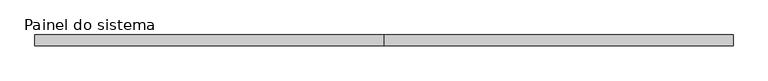
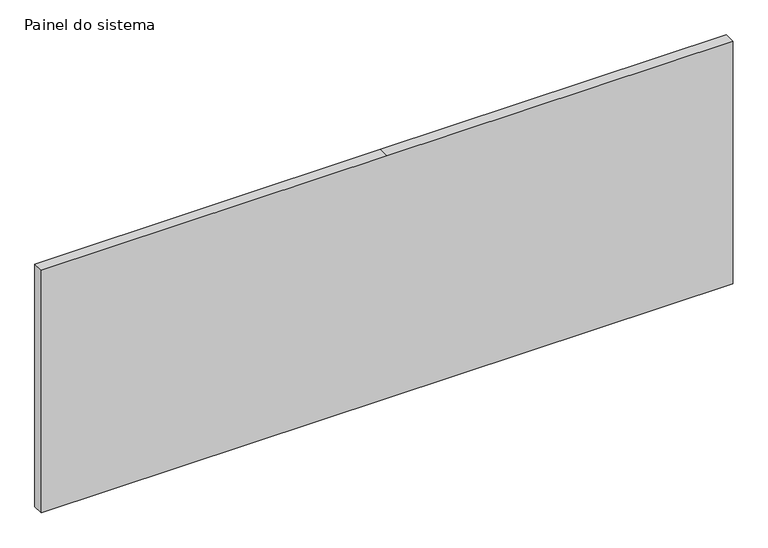
"""IFC4 building model written with IfcOpenShell, lengths in millimetres: plate geometry, Painel do sistema : Envidraçado."""

import ifcopenshell
import ifcopenshell.guid

model = None  # the IFC model being written
_history = None  # IfcOwnerHistory: only IFC2X3 demands one
_inside = {}  # id of a spatial element -> (the spatial element, [elements in it])
_under = {}  # id of a project, library or spatial element -> (it, [spatial elements below it])
_declared = {}  # id of a project -> (the project, [libraries it declares])
_typed = {}  # id of a type object -> (the type object, [elements of that type])
_made_of = {}  # id of a material, layer set ... -> (it, [elements and type objects made of it])


def new_model(schema):
    """Start an empty IFC model of exactly this schema.

    Asked for "IFC4X3", IfcOpenShell would pick the latest addendum, in which some entities
    have other attributes; the version numbers below select the first issue.
    IFC2X3 requires an IfcOwnerHistory on every rooted entity: one is made here for all.
    """
    global model, _history
    if schema == "IFC4X3":
        model = ifcopenshell.file(schema_version=(4, 3, 0, 0))
    else:
        model = ifcopenshell.file(schema=schema)
    _inside.clear()
    _under.clear()
    _declared.clear()
    _typed.clear()
    _made_of.clear()
    _history = None
    if model.schema == "IFC2X3":
        org = make("IfcOrganization", Name="unknown")
        user = make(
            "IfcPersonAndOrganization",
            ThePerson=make("IfcPerson", FamilyName="unknown"),
            TheOrganization=org,
        )
        app = make(
            "IfcApplication",
            ApplicationDeveloper=org,
            Version="unknown",
            ApplicationFullName="unknown",
            ApplicationIdentifier="unknown",
        )
        _history = make(
            "IfcOwnerHistory",
            OwningUser=user,
            OwningApplication=app,
            ChangeAction="ADDED",
            CreationDate=0,
        )
    return model


def make(cls, **values):
    """One entity of the class cls with the attributes given. An attribute that is None is left unset."""
    return model.create_entity(
        cls, **{name: value for name, value in values.items() if value is not None}
    )


def rooted(cls, **values):
    """An entity with a GlobalId (a new one), such as an element, a storey or a relation."""
    return make(cls, GlobalId=ifcopenshell.guid.new(), OwnerHistory=_history, **values)


def si_unit(unit_type, name, prefix=None):
    """IfcSIUnit, for example si_unit("LENGTHUNIT", "METRE", prefix="MILLI")."""
    return make("IfcSIUnit", UnitType=unit_type, Prefix=prefix, Name=name)


def assignment(units):
    """IfcUnitAssignment: the units of a project."""
    return None if units is None else make("IfcUnitAssignment", Units=units)


def point(xyz):
    """IfcCartesianPoint."""
    return None if xyz is None else make("IfcCartesianPoint", Coordinates=xyz)


def direction(xyz):
    """IfcDirection."""
    return None if xyz is None else make("IfcDirection", DirectionRatios=xyz)


def frame(location, z_axis=None, x_axis=None):
    """IfcAxis2Placement3D, a coordinate frame: its origin and axes. An axis left out is left unset."""
    return make(
        "IfcAxis2Placement3D",
        Location=point(location),
        Axis=direction(z_axis),
        RefDirection=direction(x_axis),
    )


def origin():
    """The frame at (0, 0, 0) with its axes left unset."""
    return frame((0.0, 0.0, 0.0))


def place(relative_to, where):
    """IfcLocalPlacement: puts the frame where relative to a parent placement (None: the world)."""
    return make(
        "IfcLocalPlacement", PlacementRelTo=relative_to, RelativePlacement=where
    )


def context(
    kind, dimensions, precision=None, world=None, true_north=None, identifier=None
):
    """IfcGeometricRepresentationContext, for example the 3D "Model" context."""
    return make(
        "IfcGeometricRepresentationContext",
        ContextIdentifier=identifier,
        ContextType=kind,
        CoordinateSpaceDimension=dimensions,
        Precision=precision,
        WorldCoordinateSystem=world,
        TrueNorth=true_north,
    )


def project(units=None, contexts=None):
    """IfcProject with its units and contexts."""
    return rooted(
        "IfcProject",
        Name="project",
        RepresentationContexts=contexts,
        UnitsInContext=assignment(units),
    )


def spatial(cls, under=None, at=None, **own):
    """A site, building, storey or space (cls), placed at a placement, below another one or the project."""
    s = rooted(cls, ObjectPlacement=at, **own)
    if under is not None:
        _under.setdefault(under.id(), (under, []))[1].append(s)
    return s


def polyline(points):
    """IfcPolyline through the points."""
    return make("IfcPolyline", Points=[point(p) for p in points])


def outline(outer, holes=None, kind="AREA"):
    """IfcArbitraryClosedProfileDef: a profile drawn as a closed curve; with holes, ...WithVoids."""
    if holes is None:
        return make("IfcArbitraryClosedProfileDef", ProfileType=kind, OuterCurve=outer)
    return make(
        "IfcArbitraryProfileDefWithVoids",
        ProfileType=kind,
        OuterCurve=outer,
        InnerCurves=holes,
    )


def extrude(swept, where, along, depth):
    """IfcExtrudedAreaSolid: the profile swept, set in the frame where, extruded along a direction by depth."""
    return make(
        "IfcExtrudedAreaSolid",
        SweptArea=swept,
        Position=where,
        ExtrudedDirection=direction(along),
        Depth=depth,
    )


def shape(context_of_items, identifier, shape_type, items):
    """IfcShapeRepresentation: the items that make up one representation, for example the "Body"."""
    return make(
        "IfcShapeRepresentation",
        ContextOfItems=context_of_items,
        RepresentationIdentifier=identifier,
        RepresentationType=shape_type,
        Items=items,
    )


def source(mapping_origin, context_of_items, identifier, shape_type, items):
    """IfcRepresentationMap: a shape defined once, which mapped items show again and again."""
    return make(
        "IfcRepresentationMap",
        MappingOrigin=mapping_origin,
        MappedRepresentation=shape(context_of_items, identifier, shape_type, items),
    )


def transform(
    local_origin,
    x_axis=None,
    y_axis=None,
    z_axis=None,
    scale=None,
    scale2=None,
    scale3=None,
    uniform=True,
):
    """IfcCartesianTransformationOperator3D, or its non-uniform kind. x_axis, y_axis, z_axis: its Axis1, 2, 3."""
    if uniform:
        return make(
            "IfcCartesianTransformationOperator3D",
            Axis1=direction(x_axis),
            Axis2=direction(y_axis),
            LocalOrigin=point(local_origin),
            Scale=scale,
            Axis3=direction(z_axis),
        )
    return make(
        "IfcCartesianTransformationOperator3DnonUniform",
        Axis1=direction(x_axis),
        Axis2=direction(y_axis),
        LocalOrigin=point(local_origin),
        Scale=scale,
        Axis3=direction(z_axis),
        Scale2=scale2,
        Scale3=scale3,
    )


def mapped(mapping_source, mapping_target):
    """IfcMappedItem: shows the shape of a source again, moved by a transform."""
    return make(
        "IfcMappedItem", MappingSource=mapping_source, MappingTarget=mapping_target
    )


def made_of(thing, what):
    """Note that an element or type object is made of a material, layer set ...; save() writes the relation."""
    if what is not None:
        _made_of.setdefault(what.id(), (what, []))[1].append(thing)
    return thing


def element(
    cls,
    number,
    at=None,
    inside=None,
    cuts=None,
    type_object=None,
    material=None,
    context=None,
    identifier="Body",
    shape_type=None,
    held_by="IfcProductDefinitionShape",
    body=None,
    shapes=None,
    **own,
):
    """One element of the class cls, such as IfcWall. Its Tag is "e" and its number.

    at: its placement. inside: the storey or other place that contains it. cuts: it is an
    opening in that element (IfcRelVoidsElement). A single representation is given by context,
    identifier, shape_type and body (its items); several are given by shapes. held_by: the class
    of the entity that holds the representations. save() writes the other relations.
    """
    e = rooted(cls, Tag="e%d" % number, ObjectPlacement=at, **own)
    if body is not None:
        shapes = [shape(context, identifier, shape_type, body)]
    if shapes is not None:
        e.Representation = make(held_by, Representations=shapes)
    if inside is not None:
        _inside.setdefault(inside.id(), (inside, []))[1].append(e)
    if cuts is not None:
        rooted(
            "IfcRelVoidsElement", RelatingBuildingElement=cuts, RelatedOpeningElement=e
        )
    if type_object is not None:
        _typed.setdefault(type_object.id(), (type_object, []))[1].append(e)
    return made_of(e, material)


def aggregate(whole, parts):
    """IfcRelAggregates: a whole, such as a stair, and the parts it consists of."""
    return rooted("IfcRelAggregates", RelatingObject=whole, RelatedObjects=parts)


def save(model, path):
    """Write the relations noted so far, then the file.

    IfcRelAggregates (storeys below a building ...), IfcRelContainedInSpatialStructure (elements
    in a storey), IfcRelDefinesByType, IfcRelAssociatesMaterial and IfcRelDeclares: one each for
    every whole, place, type object, material and project.
    """
    for whole, parts in _under.values():
        aggregate(whole, parts)
    for where, things in _inside.values():
        rooted(
            "IfcRelContainedInSpatialStructure",
            RelatedElements=things,
            RelatingStructure=where,
        )
    for kind, things in _typed.values():
        rooted("IfcRelDefinesByType", RelatedObjects=things, RelatingType=kind)
    for what, things in _made_of.values():
        rooted("IfcRelAssociatesMaterial", RelatedObjects=things, RelatingMaterial=what)
    for by, libraries in _declared.values():
        rooted("IfcRelDeclares", RelatingContext=by, RelatedDefinitions=libraries)
    model.write(path)


def painel_do_sistema_17e406c8(model_context):
    return source(origin(), model_context, "Body", "SweptSolid", [
        extrude(outline(polyline([(0.0, -795.9833332), (0.0, 0.0), (0.0, 795.9833332), (590.0, 795.9833332), (590.0, 0.0), (590.0, -795.9833332), (0.0, -795.9833332)])), frame((0.0, -49.5, 0.0), z_axis=(0.0, 1.0, 0.0), x_axis=(0.0, 0.0, 1.0)), (0.0, 0.0, 1.0), 25.0),
    ])


if __name__ == "__main__":
    model = new_model("IFC4")
    model_context = context("Model", 3, world=origin())
    ifc_project = project(units=[si_unit("LENGTHUNIT", "METRE", prefix="MILLI")], contexts=[model_context])
    site = spatial("IfcSite", under=ifc_project)
    building = spatial("IfcBuilding", under=site)
    placement = place(None, origin())
    painel_do_sistema_shape = painel_do_sistema_17e406c8(model_context)
    element("IfcPlate", 1, ObjectType="Painel do sistema : Envidraçado", at=placement, inside=building, context=model_context, shape_type="MappedRepresentation", body=[
        mapped(painel_do_sistema_shape, transform((0.0, 0.0, 0.0), x_axis=(1.0, 0.0, 0.0), y_axis=(0.0, 1.0, 0.0), z_axis=(0.0, 0.0, 1.0))),
    ])
    save(model, "model.ifc")

# Revit data of these elements
# Project information
#   Design Option = "Main Model"
#   Project Status = "Status do projeto"
#   Client Name = "JOÃO MATIAS SOARES"
#   Project Address = "RUA SÉRGIO DIAS, LOTE 30, QUADRA G, MONTE MINEIRO/MG"
#   Project Name = "CONSTRUÇÃO RESIDENCIA UNIFAMILIAR"
#   Project Number = "034/2017"
#   Zona = "ZER - 01"
#   CA Mín = "0.2"
#   CA Básico = "1"
#   CA Máx = "2"
#   TO Máx = "50"
#   Gabarito Máx = "10"
#   TP Mín = "15"
#   Área Total do Terreno = "620.00 m²"
#   Multifamiliar - Vagas Veículos/Pavto = "0"
#   Multifamiliar - Vagas Bicicletas/Pavto = "0"
#   Multifamiliar - % Vagas PNMR = "0"
#   Multifamiliar - % Vagas Motos = "0"
#   Outros - Área p/ 1 Veículo = "0.00 m²"
#   Outros - Área p/ 1 Bicicleta = "0.00 m²"
#   Outros - Área p/ 1 Utilitário = "0.00 m²"
#   Outros - % Vagas PNMR = "0"
#   Outros - % Vagas Motos = "0"
# Type "Painel do sistema : Envidraçado"
#   Construction Type Id = "GSP4R"
#   Analytic Construction = "Vidraça única Pilkington 1/8 pol"
#   Visual Light Transmittance = 0.9
#   Solar Heat Gain Coefficient = 0.86
#   Heat Transfer Coefficient (U) = 6.7069 W/(m²·K)
# Element 1 (IfcPlate, "Painel do sistema : Envidraçado")
#   Materials on its faces: ".VIDRO GENÉRICO"
# Materials
#   ".VIDRO GENÉRICO": class ".CC_VIDRO", colour RGB 0 128 192, transparency 0.9, Description = "Vidro comum", Cost = 0
